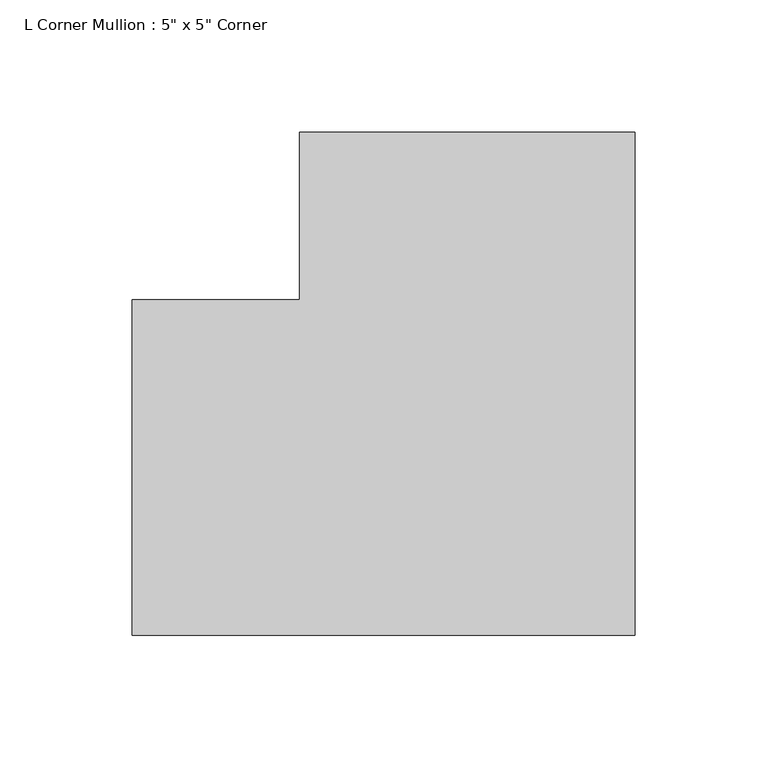
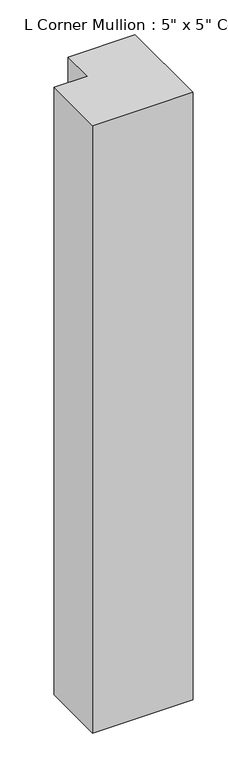
"""IFC4 building model written with IfcOpenShell, lengths in millimetres: member geometry."""

from ifc_helpers import new_model, si_unit, frame, origin, place, context, project, spatial, polyline, outline, extrude, source, transform, mapped, element, save


def member_863be36e(model_context):
    return source(origin(), model_context, "Body", "SweptSolid", [
        extrude(outline(polyline([(63.5, 127.0), (63.5, -63.5), (-127.0, -63.5), (-127.0, 63.5), (-63.5, 63.5), (-63.5, 127.0), (63.5, 127.0)])), frame((0.0, 0.0, -1219.2), z_axis=(0.0, 0.0, 1.0), x_axis=(1.0, 0.0, 0.0)), (0.0, 0.0, 1.0), 1219.2),
    ])


if __name__ == "__main__":
    model = new_model("IFC4")
    model_context = context("Model", 3, world=origin())
    ifc_project = project(units=[si_unit("LENGTHUNIT", "METRE", prefix="MILLI")], contexts=[model_context])
    site = spatial("IfcSite", under=ifc_project)
    building = spatial("IfcBuilding", under=site)
    placement = place(None, origin())
    member_shape = member_863be36e(model_context)
    element("IfcMember", 1, ObjectType="L Corner Mullion : 5\" x 5\" Corner", at=placement, inside=building, context=model_context, shape_type="MappedRepresentation", body=[
        mapped(member_shape, transform((0.0, 0.0, 0.0), x_axis=(1.0, 0.0, 0.0), y_axis=(0.0, 1.0, 0.0), z_axis=(0.0, 0.0, 1.0))),
    ])
    save(model, "model.ifc")

# Revit data of these elements
# Type "L Corner Mullion : 5\" x 5\" Corner"
#   built-in parameter 1007355 = 0.416667 (stored number, unit not read)
#   built-in parameter 1007354 = 0.416667 (stored number, unit not read)
#   built-in parameter 1007304 = 0.416667 (stored number, unit not read)
# Element 1 (IfcMember, "L Corner Mullion : 5\" x 5\" Corner")
#   Materials on its faces: "Metal - Aluminum"
# Materials
#   "Metal - Aluminum": class "Metal", colour RGB 140 140 140, transparency 0
